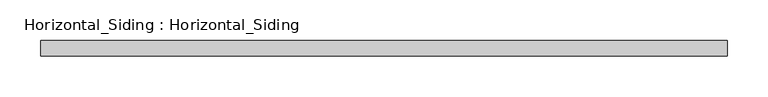
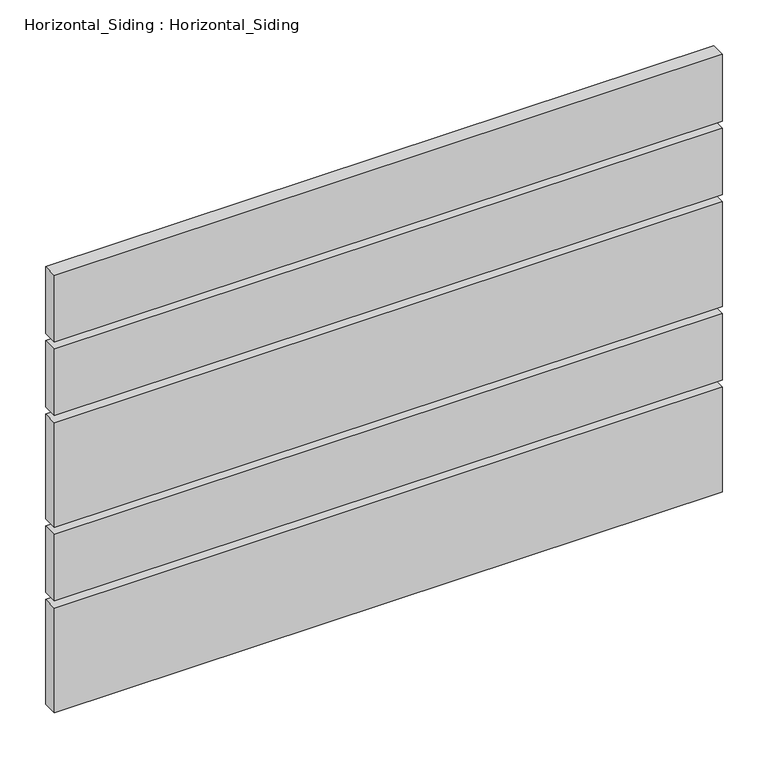
"""IFC4 building model written with IfcOpenShell, lengths in millimetres: plate geometry, Horizontal_Siding : Horizontal_Siding."""

import ifcopenshell
import ifcopenshell.guid

model = None  # the IFC model being written
_history = None  # IfcOwnerHistory: only IFC2X3 demands one
_inside = {}  # id of a spatial element -> (the spatial element, [elements in it])
_under = {}  # id of a project, library or spatial element -> (it, [spatial elements below it])
_declared = {}  # id of a project -> (the project, [libraries it declares])
_typed = {}  # id of a type object -> (the type object, [elements of that type])
_made_of = {}  # id of a material, layer set ... -> (it, [elements and type objects made of it])


def new_model(schema):
    """Start an empty IFC model of exactly this schema.

    Asked for "IFC4X3", IfcOpenShell would pick the latest addendum, in which some entities
    have other attributes; the version numbers below select the first issue.
    IFC2X3 requires an IfcOwnerHistory on every rooted entity: one is made here for all.
    """
    global model, _history
    if schema == "IFC4X3":
        model = ifcopenshell.file(schema_version=(4, 3, 0, 0))
    else:
        model = ifcopenshell.file(schema=schema)
    _inside.clear()
    _under.clear()
    _declared.clear()
    _typed.clear()
    _made_of.clear()
    _history = None
    if model.schema == "IFC2X3":
        org = make("IfcOrganization", Name="unknown")
        user = make(
            "IfcPersonAndOrganization",
            ThePerson=make("IfcPerson", FamilyName="unknown"),
            TheOrganization=org,
        )
        app = make(
            "IfcApplication",
            ApplicationDeveloper=org,
            Version="unknown",
            ApplicationFullName="unknown",
            ApplicationIdentifier="unknown",
        )
        _history = make(
            "IfcOwnerHistory",
            OwningUser=user,
            OwningApplication=app,
            ChangeAction="ADDED",
            CreationDate=0,
        )
    return model


def make(cls, **values):
    """One entity of the class cls with the attributes given. An attribute that is None is left unset."""
    return model.create_entity(
        cls, **{name: value for name, value in values.items() if value is not None}
    )


def rooted(cls, **values):
    """An entity with a GlobalId (a new one), such as an element, a storey or a relation."""
    return make(cls, GlobalId=ifcopenshell.guid.new(), OwnerHistory=_history, **values)


def si_unit(unit_type, name, prefix=None):
    """IfcSIUnit, for example si_unit("LENGTHUNIT", "METRE", prefix="MILLI")."""
    return make("IfcSIUnit", UnitType=unit_type, Prefix=prefix, Name=name)


def assignment(units):
    """IfcUnitAssignment: the units of a project."""
    return None if units is None else make("IfcUnitAssignment", Units=units)


def point(xyz):
    """IfcCartesianPoint."""
    return None if xyz is None else make("IfcCartesianPoint", Coordinates=xyz)


def direction(xyz):
    """IfcDirection."""
    return None if xyz is None else make("IfcDirection", DirectionRatios=xyz)


def frame(location, z_axis=None, x_axis=None):
    """IfcAxis2Placement3D, a coordinate frame: its origin and axes. An axis left out is left unset."""
    return make(
        "IfcAxis2Placement3D",
        Location=point(location),
        Axis=direction(z_axis),
        RefDirection=direction(x_axis),
    )


def origin():
    """The frame at (0, 0, 0) with its axes left unset."""
    return frame((0.0, 0.0, 0.0))


def place(relative_to, where):
    """IfcLocalPlacement: puts the frame where relative to a parent placement (None: the world)."""
    return make(
        "IfcLocalPlacement", PlacementRelTo=relative_to, RelativePlacement=where
    )


def context(
    kind, dimensions, precision=None, world=None, true_north=None, identifier=None
):
    """IfcGeometricRepresentationContext, for example the 3D "Model" context."""
    return make(
        "IfcGeometricRepresentationContext",
        ContextIdentifier=identifier,
        ContextType=kind,
        CoordinateSpaceDimension=dimensions,
        Precision=precision,
        WorldCoordinateSystem=world,
        TrueNorth=true_north,
    )


def project(units=None, contexts=None):
    """IfcProject with its units and contexts."""
    return rooted(
        "IfcProject",
        Name="project",
        RepresentationContexts=contexts,
        UnitsInContext=assignment(units),
    )


def spatial(cls, under=None, at=None, **own):
    """A site, building, storey or space (cls), placed at a placement, below another one or the project."""
    s = rooted(cls, ObjectPlacement=at, **own)
    if under is not None:
        _under.setdefault(under.id(), (under, []))[1].append(s)
    return s


def polyline(points):
    """IfcPolyline through the points."""
    return make("IfcPolyline", Points=[point(p) for p in points])


def outline(outer, holes=None, kind="AREA"):
    """IfcArbitraryClosedProfileDef: a profile drawn as a closed curve; with holes, ...WithVoids."""
    if holes is None:
        return make("IfcArbitraryClosedProfileDef", ProfileType=kind, OuterCurve=outer)
    return make(
        "IfcArbitraryProfileDefWithVoids",
        ProfileType=kind,
        OuterCurve=outer,
        InnerCurves=holes,
    )


def extrude(swept, where, along, depth):
    """IfcExtrudedAreaSolid: the profile swept, set in the frame where, extruded along a direction by depth."""
    return make(
        "IfcExtrudedAreaSolid",
        SweptArea=swept,
        Position=where,
        ExtrudedDirection=direction(along),
        Depth=depth,
    )


def shape(context_of_items, identifier, shape_type, items):
    """IfcShapeRepresentation: the items that make up one representation, for example the "Body"."""
    return make(
        "IfcShapeRepresentation",
        ContextOfItems=context_of_items,
        RepresentationIdentifier=identifier,
        RepresentationType=shape_type,
        Items=items,
    )


def source(mapping_origin, context_of_items, identifier, shape_type, items):
    """IfcRepresentationMap: a shape defined once, which mapped items show again and again."""
    return make(
        "IfcRepresentationMap",
        MappingOrigin=mapping_origin,
        MappedRepresentation=shape(context_of_items, identifier, shape_type, items),
    )


def transform(
    local_origin,
    x_axis=None,
    y_axis=None,
    z_axis=None,
    scale=None,
    scale2=None,
    scale3=None,
    uniform=True,
):
    """IfcCartesianTransformationOperator3D, or its non-uniform kind. x_axis, y_axis, z_axis: its Axis1, 2, 3."""
    if uniform:
        return make(
            "IfcCartesianTransformationOperator3D",
            Axis1=direction(x_axis),
            Axis2=direction(y_axis),
            LocalOrigin=point(local_origin),
            Scale=scale,
            Axis3=direction(z_axis),
        )
    return make(
        "IfcCartesianTransformationOperator3DnonUniform",
        Axis1=direction(x_axis),
        Axis2=direction(y_axis),
        LocalOrigin=point(local_origin),
        Scale=scale,
        Axis3=direction(z_axis),
        Scale2=scale2,
        Scale3=scale3,
    )


def mapped(mapping_source, mapping_target):
    """IfcMappedItem: shows the shape of a source again, moved by a transform."""
    return make(
        "IfcMappedItem", MappingSource=mapping_source, MappingTarget=mapping_target
    )


def made_of(thing, what):
    """Note that an element or type object is made of a material, layer set ...; save() writes the relation."""
    if what is not None:
        _made_of.setdefault(what.id(), (what, []))[1].append(thing)
    return thing


def element(
    cls,
    number,
    at=None,
    inside=None,
    cuts=None,
    type_object=None,
    material=None,
    context=None,
    identifier="Body",
    shape_type=None,
    held_by="IfcProductDefinitionShape",
    body=None,
    shapes=None,
    **own,
):
    """One element of the class cls, such as IfcWall. Its Tag is "e" and its number.

    at: its placement. inside: the storey or other place that contains it. cuts: it is an
    opening in that element (IfcRelVoidsElement). A single representation is given by context,
    identifier, shape_type and body (its items); several are given by shapes. held_by: the class
    of the entity that holds the representations. save() writes the other relations.
    """
    e = rooted(cls, Tag="e%d" % number, ObjectPlacement=at, **own)
    if body is not None:
        shapes = [shape(context, identifier, shape_type, body)]
    if shapes is not None:
        e.Representation = make(held_by, Representations=shapes)
    if inside is not None:
        _inside.setdefault(inside.id(), (inside, []))[1].append(e)
    if cuts is not None:
        rooted(
            "IfcRelVoidsElement", RelatingBuildingElement=cuts, RelatedOpeningElement=e
        )
    if type_object is not None:
        _typed.setdefault(type_object.id(), (type_object, []))[1].append(e)
    return made_of(e, material)


def aggregate(whole, parts):
    """IfcRelAggregates: a whole, such as a stair, and the parts it consists of."""
    return rooted("IfcRelAggregates", RelatingObject=whole, RelatedObjects=parts)


def save(model, path):
    """Write the relations noted so far, then the file.

    IfcRelAggregates (storeys below a building ...), IfcRelContainedInSpatialStructure (elements
    in a storey), IfcRelDefinesByType, IfcRelAssociatesMaterial and IfcRelDeclares: one each for
    every whole, place, type object, material and project.
    """
    for whole, parts in _under.values():
        aggregate(whole, parts)
    for where, things in _inside.values():
        rooted(
            "IfcRelContainedInSpatialStructure",
            RelatedElements=things,
            RelatingStructure=where,
        )
    for kind, things in _typed.values():
        rooted("IfcRelDefinesByType", RelatedObjects=things, RelatingType=kind)
    for what, things in _made_of.values():
        rooted("IfcRelAssociatesMaterial", RelatedObjects=things, RelatingMaterial=what)
    for by, libraries in _declared.values():
        rooted("IfcRelDeclares", RelatingContext=by, RelatedDefinitions=libraries)
    model.write(path)


def horizontal_siding_horizontal_siding_d6c4737b(model_context):
    return source(origin(), model_context, "Body", "SweptSolid", [
        extrude(outline(polyline([(421.48125, -19.05), (-421.48125, -19.05), (-421.48125, 0.0), (421.48125, 0.0), (421.48125, -19.05)])), frame((0.0, 0.0, 9.525), z_axis=(0.0, 0.0, 1.0), x_axis=(1.0, 0.0, 0.0)), (0.0, 0.0, 1.0), 139.7),
        extrude(outline(polyline([(421.48125, -19.05), (-421.48125, -19.05), (-421.48125, 0.0), (421.48125, 0.0), (421.48125, -19.05)])), frame((0.0, 0.0, 158.75), z_axis=(0.0, 0.0, 1.0), x_axis=(1.0, 0.0, 0.0)), (0.0, 0.0, 1.0), 88.9),
        extrude(outline(polyline([(421.48125, -19.05), (-421.48125, -19.05), (-421.48125, 0.0), (421.48125, 0.0), (421.48125, -19.05)])), frame((0.0, 0.0, 257.175), z_axis=(0.0, 0.0, 1.0), x_axis=(1.0, 0.0, 0.0)), (0.0, 0.0, 1.0), 139.7),
        extrude(outline(polyline([(421.48125, -19.05), (-421.48125, -19.05), (-421.48125, 0.0), (421.48125, 0.0), (421.48125, -19.05)])), frame((0.0, 0.0, 406.4), z_axis=(0.0, 0.0, 1.0), x_axis=(1.0, 0.0, 0.0)), (0.0, 0.0, 1.0), 88.9),
        extrude(outline(polyline([(421.48125, -19.05), (-421.48125, -19.05), (-421.48125, 0.0), (421.48125, 0.0), (421.48125, -19.05)])), frame((0.0, 0.0, 504.825), z_axis=(0.0, 0.0, 1.0), x_axis=(1.0, 0.0, 0.0)), (0.0, 0.0, 1.0), 88.9),
    ])


if __name__ == "__main__":
    model = new_model("IFC4")
    model_context = context("Model", 3, world=origin())
    ifc_project = project(units=[si_unit("LENGTHUNIT", "METRE", prefix="MILLI")], contexts=[model_context])
    site = spatial("IfcSite", under=ifc_project)
    building = spatial("IfcBuilding", under=site)
    placement = place(None, origin())
    horizontal_siding_horizontal_siding_shape = horizontal_siding_horizontal_siding_d6c4737b(model_context)
    element("IfcPlate", 1, ObjectType="Horizontal_Siding : Horizontal_Siding", at=placement, inside=building, context=model_context, shape_type="MappedRepresentation", body=[
        mapped(horizontal_siding_horizontal_siding_shape, transform((0.0, 0.0, 0.0), x_axis=(1.0, 0.0, 0.0), y_axis=(0.0, 1.0, 0.0), z_axis=(0.0, 0.0, 1.0))),
    ])
    save(model, "model.ifc")

# Revit data of these elements
# Type "Horizontal_Siding : Horizontal_Siding"
#   Type Mark = "OUT"
#   Analytic Construction = "<None>"
#   extend = 0' - 2 3/4"
#   Width_2 = 0' - 3 1/2"
#   Width_1 = 0' - 5 1/2"
#   Gap = 0' - 0 3/8"
#   Plank Material = SLOTTED WOOD FENCE (THERMALLY MODIFIED WOOD: ARBOR WOOD)\n(EXTERIOR STAIN : PENOFIN VERDE EXT. STAIN - COLOR: CEDAR)
# Element 1 (IfcPlate, "Horizontal_Siding : Horizontal_Siding")
#   Materials on its faces: "SLOTTED WOOD FENCE (THERMALLY MODIFIED WOOD: ARBOR WOOD)\n(EXTERIOR STAIN : PENOFIN VERDE EXT. STAIN - COLOR: CEDAR)"
# Materials
#   "SLOTTED WOOD FENCE (THERMALLY MODIFIED WOOD: ARBOR WOOD)\n(EXTERIOR STAIN : PENOFIN VERDE EXT. STAIN - COLOR: CEDAR)": class "Wood", colour RGB 164 134 123, transparency 0, Description = "Pinus Echinata", Cost = 0
